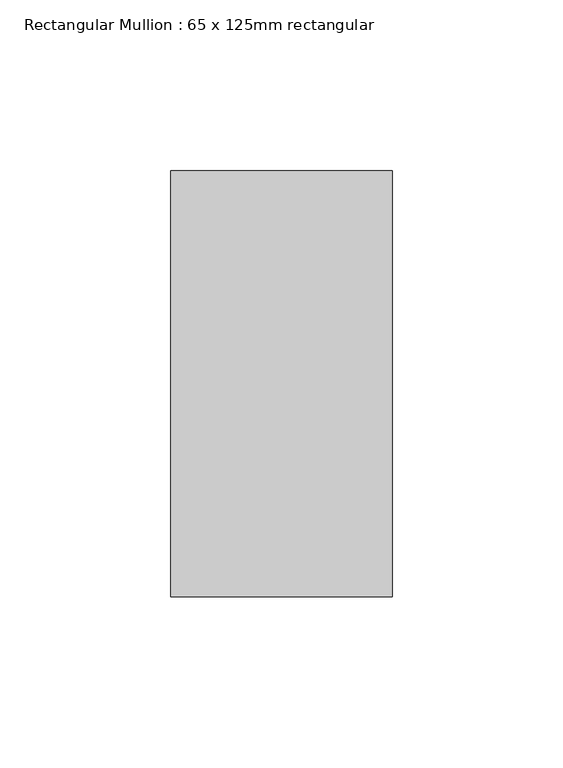
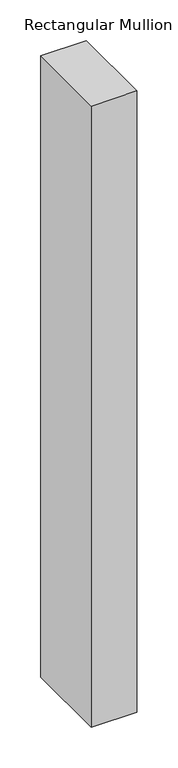
"""IFC4 building model written with IfcOpenShell, lengths in millimetres: member geometry, Rectangular Mullion : 65 x 125mm rectangular."""

from ifc_helpers import new_model, si_unit, frame, origin, place, context, project, spatial, polyline, outline, extrude, source, transform, mapped, element, save


def rectangular_mullion_65_x_125mm_rectangular_1b57746c(model_context):
    return source(origin(), model_context, "Body", "SweptSolid", [
        extrude(outline(polyline([(0.0, 62.5), (0.0, -62.5), (-65.0, -62.5), (-65.0, 62.5), (0.0, 62.5)])), frame((0.0, 0.0, -935.0), z_axis=(0.0, 0.0, 1.0), x_axis=(1.0, 0.0, 0.0)), (0.0, 0.0, 1.0), 935.0),
    ])


if __name__ == "__main__":
    model = new_model("IFC4")
    model_context = context("Model", 3, world=origin())
    ifc_project = project(units=[si_unit("LENGTHUNIT", "METRE", prefix="MILLI")], contexts=[model_context])
    site = spatial("IfcSite", under=ifc_project)
    building = spatial("IfcBuilding", under=site)
    placement = place(None, origin())
    rectangular_mullion_65_x_125mm_rectangular_shape = rectangular_mullion_65_x_125mm_rectangular_1b57746c(model_context)
    element("IfcMember", 1, ObjectType="Rectangular Mullion : 65 x 125mm rectangular", at=placement, inside=building, context=model_context, shape_type="MappedRepresentation", body=[
        mapped(rectangular_mullion_65_x_125mm_rectangular_shape, transform((0.0, 0.0, 0.0), x_axis=(1.0, 0.0, 0.0), y_axis=(0.0, 1.0, 0.0), z_axis=(0.0, 0.0, 1.0))),
    ])
    save(model, "model.ifc")

# Revit data of these elements
# Type "Rectangular Mullion : 65 x 125mm rectangular"
#   built-in parameter 1007304 = 0.410105 (stored number, unit not read)
#   built-in parameter 1007301 = 0.106627 (stored number, unit not read)
#   built-in parameter 1007300 = 0.106627 (stored number, unit not read)
# Element 1 (IfcMember, "Rectangular Mullion : 65 x 125mm rectangular")
#   Materials on its faces: "Aluminum"
# Materials
#   "Aluminum": class "Metal", colour RGB 244 245 246, transparency 0, Description = "Aluminum 6061", Cost = 0
